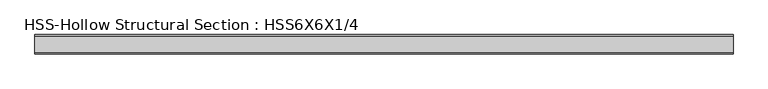
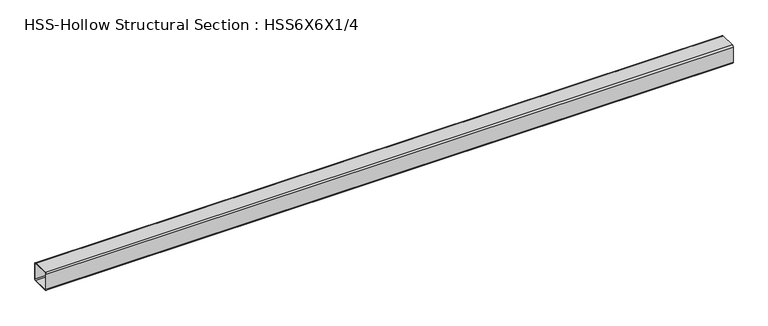
"""IFC4 building model written with IfcOpenShell, lengths in millimetres: beam geometry, HSS-Hollow Structural Section : HSS6X6X1/4."""

import ifcopenshell
import ifcopenshell.guid

model = None  # the IFC model being written
_history = None  # IfcOwnerHistory: only IFC2X3 demands one
_inside = {}  # id of a spatial element -> (the spatial element, [elements in it])
_under = {}  # id of a project, library or spatial element -> (it, [spatial elements below it])
_declared = {}  # id of a project -> (the project, [libraries it declares])
_typed = {}  # id of a type object -> (the type object, [elements of that type])
_made_of = {}  # id of a material, layer set ... -> (it, [elements and type objects made of it])


def new_model(schema):
    """Start an empty IFC model of exactly this schema.

    Asked for "IFC4X3", IfcOpenShell would pick the latest addendum, in which some entities
    have other attributes; the version numbers below select the first issue.
    IFC2X3 requires an IfcOwnerHistory on every rooted entity: one is made here for all.
    """
    global model, _history
    if schema == "IFC4X3":
        model = ifcopenshell.file(schema_version=(4, 3, 0, 0))
    else:
        model = ifcopenshell.file(schema=schema)
    _inside.clear()
    _under.clear()
    _declared.clear()
    _typed.clear()
    _made_of.clear()
    _history = None
    if model.schema == "IFC2X3":
        org = make("IfcOrganization", Name="unknown")
        user = make(
            "IfcPersonAndOrganization",
            ThePerson=make("IfcPerson", FamilyName="unknown"),
            TheOrganization=org,
        )
        app = make(
            "IfcApplication",
            ApplicationDeveloper=org,
            Version="unknown",
            ApplicationFullName="unknown",
            ApplicationIdentifier="unknown",
        )
        _history = make(
            "IfcOwnerHistory",
            OwningUser=user,
            OwningApplication=app,
            ChangeAction="ADDED",
            CreationDate=0,
        )
    return model


def make(cls, **values):
    """One entity of the class cls with the attributes given. An attribute that is None is left unset."""
    return model.create_entity(
        cls, **{name: value for name, value in values.items() if value is not None}
    )


def rooted(cls, **values):
    """An entity with a GlobalId (a new one), such as an element, a storey or a relation."""
    return make(cls, GlobalId=ifcopenshell.guid.new(), OwnerHistory=_history, **values)


def si_unit(unit_type, name, prefix=None):
    """IfcSIUnit, for example si_unit("LENGTHUNIT", "METRE", prefix="MILLI")."""
    return make("IfcSIUnit", UnitType=unit_type, Prefix=prefix, Name=name)


def assignment(units):
    """IfcUnitAssignment: the units of a project."""
    return None if units is None else make("IfcUnitAssignment", Units=units)


def point(xyz):
    """IfcCartesianPoint."""
    return None if xyz is None else make("IfcCartesianPoint", Coordinates=xyz)


def direction(xyz):
    """IfcDirection."""
    return None if xyz is None else make("IfcDirection", DirectionRatios=xyz)


def frame(location, z_axis=None, x_axis=None):
    """IfcAxis2Placement3D, a coordinate frame: its origin and axes. An axis left out is left unset."""
    return make(
        "IfcAxis2Placement3D",
        Location=point(location),
        Axis=direction(z_axis),
        RefDirection=direction(x_axis),
    )


def frame_2d(location, x_axis=None):
    """IfcAxis2Placement2D, a coordinate frame in the plane: its origin and x axis."""
    return make(
        "IfcAxis2Placement2D", Location=point(location), RefDirection=direction(x_axis)
    )


def origin():
    """The frame at (0, 0, 0) with its axes left unset."""
    return frame((0.0, 0.0, 0.0))


def place(relative_to, where):
    """IfcLocalPlacement: puts the frame where relative to a parent placement (None: the world)."""
    return make(
        "IfcLocalPlacement", PlacementRelTo=relative_to, RelativePlacement=where
    )


def context(
    kind, dimensions, precision=None, world=None, true_north=None, identifier=None
):
    """IfcGeometricRepresentationContext, for example the 3D "Model" context."""
    return make(
        "IfcGeometricRepresentationContext",
        ContextIdentifier=identifier,
        ContextType=kind,
        CoordinateSpaceDimension=dimensions,
        Precision=precision,
        WorldCoordinateSystem=world,
        TrueNorth=true_north,
    )


def project(units=None, contexts=None):
    """IfcProject with its units and contexts."""
    return rooted(
        "IfcProject",
        Name="project",
        RepresentationContexts=contexts,
        UnitsInContext=assignment(units),
    )


def spatial(cls, under=None, at=None, **own):
    """A site, building, storey or space (cls), placed at a placement, below another one or the project."""
    s = rooted(cls, ObjectPlacement=at, **own)
    if under is not None:
        _under.setdefault(under.id(), (under, []))[1].append(s)
    return s


def polyline(points):
    """IfcPolyline through the points."""
    return make("IfcPolyline", Points=[point(p) for p in points])


def circle_curve(where, radius):
    """IfcCircle in the frame where."""
    return make("IfcCircle", Position=where, Radius=radius)


def trimmed(basis, trim1, trim2, sense, master):
    """IfcTrimmedCurve: the piece of a basis curve between two trims."""
    return make(
        "IfcTrimmedCurve",
        BasisCurve=basis,
        Trim1=trim1,
        Trim2=trim2,
        SenseAgreement=sense,
        MasterRepresentation=master,
    )


def segment(curve, same_sense, transition):
    """IfcCompositeCurveSegment."""
    return make(
        "IfcCompositeCurveSegment",
        Transition=transition,
        SameSense=same_sense,
        ParentCurve=curve,
    )


def composite_curve(segments, self_intersect=None):
    """IfcCompositeCurve: segments joined end to end."""
    return make("IfcCompositeCurve", Segments=segments, SelfIntersect=self_intersect)


def outline(outer, holes=None, kind="AREA"):
    """IfcArbitraryClosedProfileDef: a profile drawn as a closed curve; with holes, ...WithVoids."""
    if holes is None:
        return make("IfcArbitraryClosedProfileDef", ProfileType=kind, OuterCurve=outer)
    return make(
        "IfcArbitraryProfileDefWithVoids",
        ProfileType=kind,
        OuterCurve=outer,
        InnerCurves=holes,
    )


def extrude(swept, where, along, depth):
    """IfcExtrudedAreaSolid: the profile swept, set in the frame where, extruded along a direction by depth."""
    return make(
        "IfcExtrudedAreaSolid",
        SweptArea=swept,
        Position=where,
        ExtrudedDirection=direction(along),
        Depth=depth,
    )


def shape(context_of_items, identifier, shape_type, items):
    """IfcShapeRepresentation: the items that make up one representation, for example the "Body"."""
    return make(
        "IfcShapeRepresentation",
        ContextOfItems=context_of_items,
        RepresentationIdentifier=identifier,
        RepresentationType=shape_type,
        Items=items,
    )


def source(mapping_origin, context_of_items, identifier, shape_type, items):
    """IfcRepresentationMap: a shape defined once, which mapped items show again and again."""
    return make(
        "IfcRepresentationMap",
        MappingOrigin=mapping_origin,
        MappedRepresentation=shape(context_of_items, identifier, shape_type, items),
    )


def transform(
    local_origin,
    x_axis=None,
    y_axis=None,
    z_axis=None,
    scale=None,
    scale2=None,
    scale3=None,
    uniform=True,
):
    """IfcCartesianTransformationOperator3D, or its non-uniform kind. x_axis, y_axis, z_axis: its Axis1, 2, 3."""
    if uniform:
        return make(
            "IfcCartesianTransformationOperator3D",
            Axis1=direction(x_axis),
            Axis2=direction(y_axis),
            LocalOrigin=point(local_origin),
            Scale=scale,
            Axis3=direction(z_axis),
        )
    return make(
        "IfcCartesianTransformationOperator3DnonUniform",
        Axis1=direction(x_axis),
        Axis2=direction(y_axis),
        LocalOrigin=point(local_origin),
        Scale=scale,
        Axis3=direction(z_axis),
        Scale2=scale2,
        Scale3=scale3,
    )


def mapped(mapping_source, mapping_target):
    """IfcMappedItem: shows the shape of a source again, moved by a transform."""
    return make(
        "IfcMappedItem", MappingSource=mapping_source, MappingTarget=mapping_target
    )


def made_of(thing, what):
    """Note that an element or type object is made of a material, layer set ...; save() writes the relation."""
    if what is not None:
        _made_of.setdefault(what.id(), (what, []))[1].append(thing)
    return thing


def element(
    cls,
    number,
    at=None,
    inside=None,
    cuts=None,
    type_object=None,
    material=None,
    context=None,
    identifier="Body",
    shape_type=None,
    held_by="IfcProductDefinitionShape",
    body=None,
    shapes=None,
    **own,
):
    """One element of the class cls, such as IfcWall. Its Tag is "e" and its number.

    at: its placement. inside: the storey or other place that contains it. cuts: it is an
    opening in that element (IfcRelVoidsElement). A single representation is given by context,
    identifier, shape_type and body (its items); several are given by shapes. held_by: the class
    of the entity that holds the representations. save() writes the other relations.
    """
    e = rooted(cls, Tag="e%d" % number, ObjectPlacement=at, **own)
    if body is not None:
        shapes = [shape(context, identifier, shape_type, body)]
    if shapes is not None:
        e.Representation = make(held_by, Representations=shapes)
    if inside is not None:
        _inside.setdefault(inside.id(), (inside, []))[1].append(e)
    if cuts is not None:
        rooted(
            "IfcRelVoidsElement", RelatingBuildingElement=cuts, RelatedOpeningElement=e
        )
    if type_object is not None:
        _typed.setdefault(type_object.id(), (type_object, []))[1].append(e)
    return made_of(e, material)


def aggregate(whole, parts):
    """IfcRelAggregates: a whole, such as a stair, and the parts it consists of."""
    return rooted("IfcRelAggregates", RelatingObject=whole, RelatedObjects=parts)


def save(model, path):
    """Write the relations noted so far, then the file.

    IfcRelAggregates (storeys below a building ...), IfcRelContainedInSpatialStructure (elements
    in a storey), IfcRelDefinesByType, IfcRelAssociatesMaterial and IfcRelDeclares: one each for
    every whole, place, type object, material and project.
    """
    for whole, parts in _under.values():
        aggregate(whole, parts)
    for where, things in _inside.values():
        rooted(
            "IfcRelContainedInSpatialStructure",
            RelatedElements=things,
            RelatingStructure=where,
        )
    for kind, things in _typed.values():
        rooted("IfcRelDefinesByType", RelatedObjects=things, RelatingType=kind)
    for what, things in _made_of.values():
        rooted("IfcRelAssociatesMaterial", RelatedObjects=things, RelatingMaterial=what)
    for by, libraries in _declared.values():
        rooted("IfcRelDeclares", RelatingContext=by, RelatedDefinitions=libraries)
    model.write(path)


def hss_hollow_structural_section_hss6x6x1_4_f83ef3ea(model_context):
    return source(origin(), model_context, "Body", "SweptSolid", [
        extrude(outline(composite_curve([segment(polyline([(76.2, 64.3636), (76.2, -64.3636)]), True, "CONTINUOUS"), segment(trimmed(circle_curve(frame_2d((64.3636, -64.3636)), 11.8364), [point((76.2, -64.3636))], [point((64.3636, -76.2))], False, "CARTESIAN"), True, "CONTINUOUS"), segment(polyline([(64.3636, -76.2), (-64.3636, -76.2)]), True, "CONTINUOUS"), segment(trimmed(circle_curve(frame_2d((-64.3636, -64.3636)), 11.8364), [point((-64.3636, -76.2))], [point((-76.2, -64.3636))], False, "CARTESIAN"), True, "CONTINUOUS"), segment(polyline([(-76.2, -64.3636), (-76.2, 64.3636)]), True, "CONTINUOUS"), segment(trimmed(circle_curve(frame_2d((-64.3636, 64.3636)), 11.8364), [point((-76.2, 64.3636))], [point((-64.3636, 76.2))], False, "CARTESIAN"), True, "CONTINUOUS"), segment(polyline([(-64.3636, 76.2), (64.3636, 76.2)]), True, "CONTINUOUS"), segment(trimmed(circle_curve(frame_2d((64.3636, 64.3636)), 11.8364), [point((64.3636, 76.2))], [point((76.2, 64.3636))], False, "CARTESIAN"), True, "CONTINUOUS")], self_intersect=False), holes=[composite_curve([segment(trimmed(circle_curve(frame_2d((-64.3636, 64.3636)), 5.9182), [point((-64.3636, 70.2818))], [point((-70.2818, 64.3636))], True, "CARTESIAN"), True, "CONTINUOUS"), segment(polyline([(-70.2818, 64.3636), (-70.2818, -64.3636)]), True, "CONTINUOUS"), segment(trimmed(circle_curve(frame_2d((-64.3636, -64.3636)), 5.9182), [point((-70.2818, -64.3636))], [point((-64.3636, -70.2818))], True, "CARTESIAN"), True, "CONTINUOUS"), segment(polyline([(-64.3636, -70.2818), (64.3636, -70.2818)]), True, "CONTINUOUS"), segment(trimmed(circle_curve(frame_2d((64.3636, -64.3636)), 5.9182), [point((64.3636, -70.2818))], [point((70.2818, -64.3636))], True, "CARTESIAN"), True, "CONTINUOUS"), segment(polyline([(70.2818, -64.3636), (70.2818, 64.3636)]), True, "CONTINUOUS"), segment(trimmed(circle_curve(frame_2d((64.3636, 64.3636)), 5.9182), [point((70.2818, 64.3636))], [point((64.3636, 70.2818))], True, "CARTESIAN"), True, "CONTINUOUS"), segment(polyline([(64.3636, 70.2818), (-64.3636, 70.2818)]), True, "CONTINUOUS")], self_intersect=False)]), frame((-2751.100302, 0.0, 0.0), z_axis=(1.0, 0.0, 0.0), x_axis=(0.0, 1.0, 0.0)), (0.0, 0.0, 1.0), 5507.000302),
    ])


if __name__ == "__main__":
    model = new_model("IFC4")
    model_context = context("Model", 3, world=origin())
    ifc_project = project(units=[si_unit("LENGTHUNIT", "METRE", prefix="MILLI")], contexts=[model_context])
    site = spatial("IfcSite", under=ifc_project)
    building = spatial("IfcBuilding", under=site)
    placement = place(None, origin())
    hss_hollow_structural_section_hss6x6x1_4_shape = hss_hollow_structural_section_hss6x6x1_4_f83ef3ea(model_context)
    element("IfcBeam", 1, ObjectType="HSS-Hollow Structural Section : HSS6X6X1/4", at=placement, inside=building, context=model_context, shape_type="MappedRepresentation", body=[
        mapped(hss_hollow_structural_section_hss6x6x1_4_shape, transform((0.0, 0.0, 0.0), x_axis=(1.0, 0.0, 0.0), y_axis=(0.0, 1.0, 0.0), z_axis=(0.0, 0.0, 1.0))),
    ])
    save(model, "model.ifc")

# Revit data of these elements
# Type "HSS-Hollow Structural Section : HSS6X6X1/4"
#   Assembly Code = "B10"
#   Shape = "Square"
#   W = 19
#   Ht = 0' - 6"
#   Length [instance default] = 5' - 0"
#   b = 0' - 6"
#   kr = 0' - 0.466"
#   t = 0' - 0.233"
#   A = 0.0363889 SF
#   Structural Material [instance default] = Steel ASTM A500, Grade B, Rectangular and Square
# Element 1 (IfcBeam, "HSS-Hollow Structural Section : HSS6X6X1/4")
#   Materials on its faces: "Steel ASTM A500, Grade B, Rectangular and Square"
# Materials
#   "Steel ASTM A500, Grade B, Rectangular and Square": class "Metal", colour RGB 199 199 199, transparency 0, Description = "Carbon steel", Cost = 0
